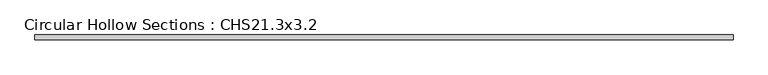
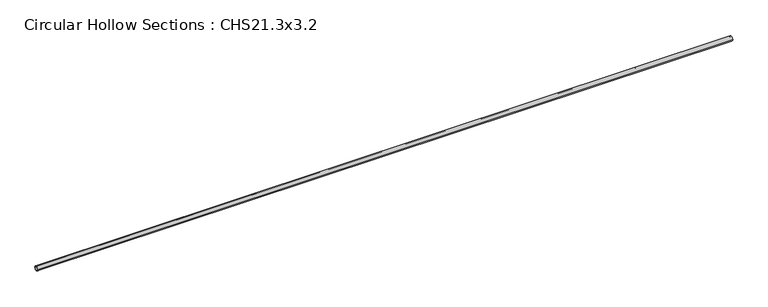
"""IFC4 building model written with IfcOpenShell, lengths in millimetres: member geometry, Circular Hollow Sections : CHS21.3x3.2."""

from ifc_helpers import new_model, si_unit, point, frame, origin, origin_2d, place, context, project, spatial, circle_curve, trimmed, segment, composite_curve, outline, extrude, source, transform, mapped, element, save


def circular_hollow_sections_chs21_3x3_2_397a7a56(model_context):
    return source(origin(), model_context, "Body", "SweptSolid", [
        extrude(outline(composite_curve([segment(trimmed(circle_curve(origin_2d(), 10.65), [point((-10.65, 0.0))], [point((10.65, 0.0))], False, "CARTESIAN"), True, "CONTINUOUS"), segment(trimmed(circle_curve(origin_2d(), 10.65), [point((10.65, 0.0))], [point((-10.65, 0.0))], False, "CARTESIAN"), True, "CONTINUOUS")], self_intersect=False), holes=[composite_curve([segment(trimmed(circle_curve(origin_2d(), 7.45), [point((7.45, 0.0))], [point((-7.45, 0.0))], True, "CARTESIAN"), True, "CONTINUOUS"), segment(trimmed(circle_curve(origin_2d(), 7.45), [point((-7.45, 0.0))], [point((7.45, 0.0))], True, "CARTESIAN"), True, "CONTINUOUS")], self_intersect=False)]), frame((-1483.85, 0.0, 0.0), z_axis=(1.0, 0.0, 0.0), x_axis=(0.0, 1.0, 0.0)), (0.0, 0.0, 1.0), 3172.9),
    ])


if __name__ == "__main__":
    model = new_model("IFC4")
    model_context = context("Model", 3, world=origin())
    ifc_project = project(units=[si_unit("LENGTHUNIT", "METRE", prefix="MILLI")], contexts=[model_context])
    site = spatial("IfcSite", under=ifc_project)
    building = spatial("IfcBuilding", under=site)
    placement = place(None, origin())
    circular_hollow_sections_chs21_3x3_2_shape = circular_hollow_sections_chs21_3x3_2_397a7a56(model_context)
    element("IfcMember", 1, ObjectType="Circular Hollow Sections : CHS21.3x3.2", at=placement, inside=building, context=model_context, shape_type="MappedRepresentation", body=[
        mapped(circular_hollow_sections_chs21_3x3_2_shape, transform((0.0, 0.0, 0.0), x_axis=(1.0, 0.0, 0.0), y_axis=(0.0, 1.0, 0.0), z_axis=(0.0, 0.0, 1.0))),
    ])
    save(model, "model.ifc")

# Revit data of these elements
# Type "Circular Hollow Sections : CHS21.3x3.2"
#   Section Name Key = "Ch21.3x3.2"
#   Wall Nominal Thickness = 0.32 cm
#   Wall Design Thickness = 0.32 cm
#   Torsional Moment of Inertia = 1.54 cm⁴
#   Torsional Modulus = 1.44 cm³
#   Section Area = 1.82 cm²
#   Plastic Modulus strong axis = 1.06 cm³
#   Perimeter = 0.067 m²/m
#   Nominal Weight = 1.42999 kgf/m
#   Moment of Inertia strong axis = 0.768 cm⁴
#   Length [instance default] = 1500 mm
#   Elastic Modulus strong axis = 0.722 cm³
#   Diameter = 2.13 cm
#   Centroid Vertical = 1.065 cm
#   Centroid Horizontal = 1.065 cm
#   Structural Material [instance default] = Metal - Steel 50-355
#   Type Comments = ""
#   Assembly Code = ""
# Element 1 (IfcMember, "Circular Hollow Sections : CHS21.3x3.2")
#   Structural Material = Metal - Steel 43-275
#   Materials on its faces: "Metal - Steel 43-275"
# Materials
#   "Metal - Steel 50-355": class "Metal", colour RGB 247 247 247, transparency 0, Cost = 0
#   "Metal - Steel 43-275": class "Metal", colour RGB 247 247 247, transparency 0, Cost = 0
